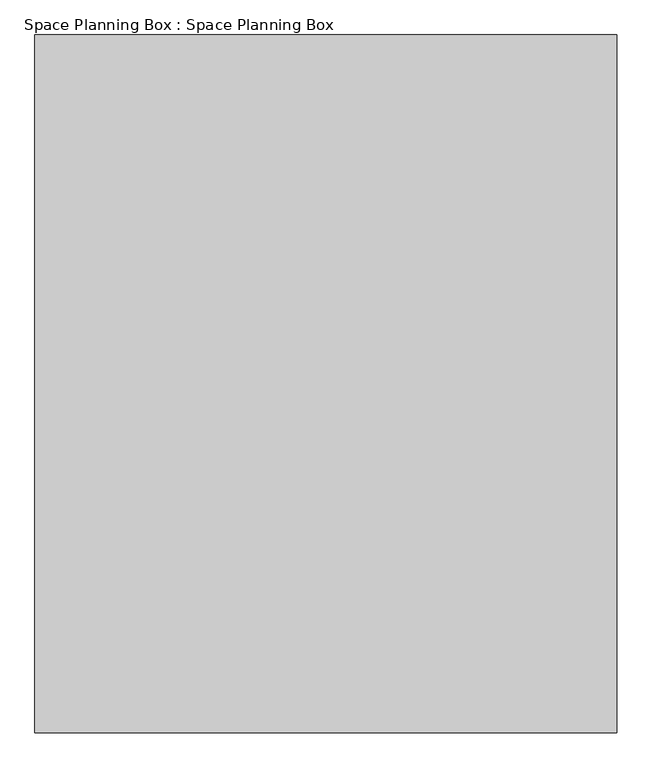
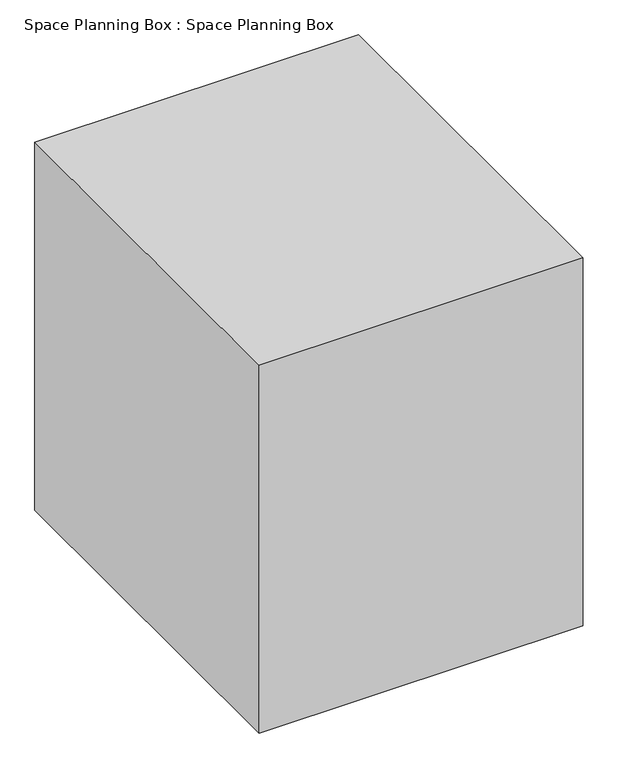
"""IFC4 building model written with IfcOpenShell, lengths in millimetres: proxy geometry, Space Planning Box : Space Planning Box."""

from ifc_helpers import new_model, si_unit, origin, origin_with_axes, place, context, project, spatial, polyline, outline, extrude, source, transform, mapped, element, save


def space_planning_box_space_planning_box_44ef6168(model_context):
    return source(origin(), model_context, "Body", "SweptSolid", [
        extrude(outline(polyline([(2500.0, 3000.0), (2500.0, -3000.0), (-2500.0, -3000.0), (-2500.0, 3000.0), (2500.0, 3000.0)])), origin_with_axes(), (0.0, 0.0, 1.0), 6000.0),
    ])


if __name__ == "__main__":
    model = new_model("IFC4")
    model_context = context("Model", 3, world=origin())
    ifc_project = project(units=[si_unit("LENGTHUNIT", "METRE", prefix="MILLI")], contexts=[model_context])
    site = spatial("IfcSite", under=ifc_project)
    building = spatial("IfcBuilding", under=site)
    placement = place(None, origin())
    space_planning_box_space_planning_box_shape = space_planning_box_space_planning_box_44ef6168(model_context)
    element("IfcBuildingElementProxy", 1, Name="Space Planning Box : Space Planning Box", ObjectType="Space Planning Box : Space Planning Box", at=placement, inside=building, context=model_context, shape_type="MappedRepresentation", body=[
        mapped(space_planning_box_space_planning_box_shape, transform((0.0, 0.0, 0.0), x_axis=(1.0, 0.0, 0.0), y_axis=(0.0, 1.0, 0.0), z_axis=(0.0, 0.0, 1.0))),
    ])
    save(model, "model.ifc")

# Revit data of these elements
# Type "Space Planning Box : Space Planning Box"
#   Type Comments = "..."
#   Room Name [instance default] = "?"
#   Assembly Code = "..."
#   Width [instance default] = 1524 mm
#   Program Area [instance default] = 0 m²
#   Length [instance default] = 1524 mm
#   Height [instance default] = 1524 mm
#   Area [instance default] = 2.32258 m²
#   Fill Color [instance default] = Cyan
#   Default Elevation = 0
# Element 1 (IfcBuildingElementProxy, "Space Planning Box : Space Planning Box")
#   Room Name = "Document Room"
#   Width = 5000 mm
#   Program Area = 48 m²
#   Length = 6000 mm
#   Height = 6000 mm
#   Area = 30 m²
#   Fill Color = Lavender
#   Materials on its faces: "Lavender"
# Materials
#   "Cyan": class "Generic", colour RGB 0 255 255, transparency 0.2, Cost = 0
#   "Lavender": class "Generic", colour RGB 186 85 211, transparency 0.2, Cost = 0
